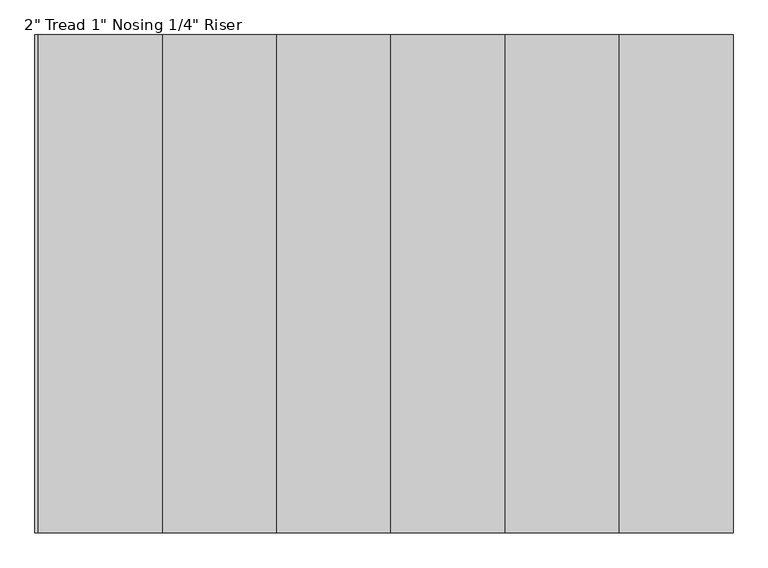
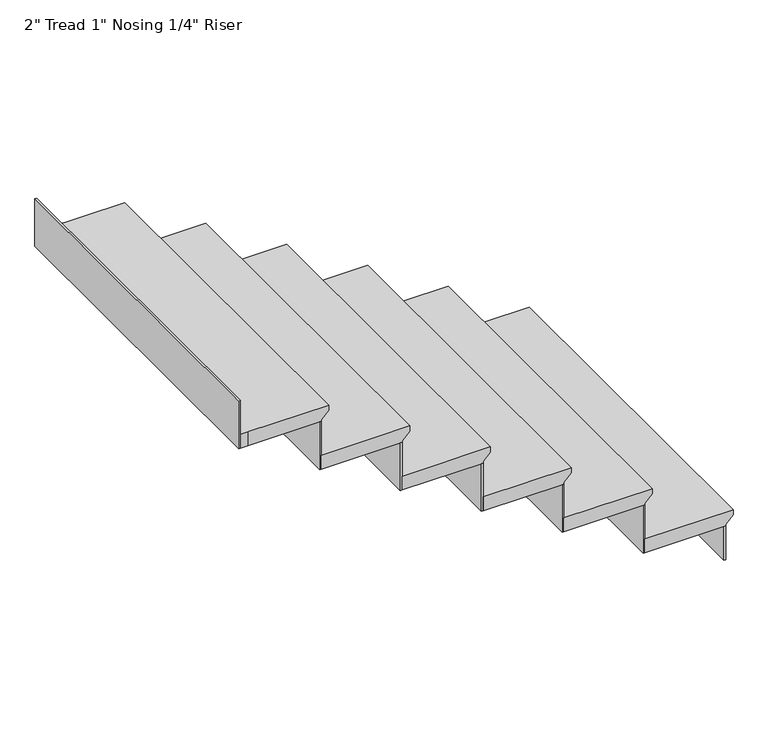
"""IFC4 building model written with IfcOpenShell, lengths in millimetres: stair flight geometry."""

import ifcopenshell
import ifcopenshell.guid

model = None  # the IFC model being written
_history = None  # IfcOwnerHistory: only IFC2X3 demands one
_inside = {}  # id of a spatial element -> (the spatial element, [elements in it])
_under = {}  # id of a project, library or spatial element -> (it, [spatial elements below it])
_declared = {}  # id of a project -> (the project, [libraries it declares])
_typed = {}  # id of a type object -> (the type object, [elements of that type])
_made_of = {}  # id of a material, layer set ... -> (it, [elements and type objects made of it])


def new_model(schema):
    """Start an empty IFC model of exactly this schema.

    Asked for "IFC4X3", IfcOpenShell would pick the latest addendum, in which some entities
    have other attributes; the version numbers below select the first issue.
    IFC2X3 requires an IfcOwnerHistory on every rooted entity: one is made here for all.
    """
    global model, _history
    if schema == "IFC4X3":
        model = ifcopenshell.file(schema_version=(4, 3, 0, 0))
    else:
        model = ifcopenshell.file(schema=schema)
    _inside.clear()
    _under.clear()
    _declared.clear()
    _typed.clear()
    _made_of.clear()
    _history = None
    if model.schema == "IFC2X3":
        org = make("IfcOrganization", Name="unknown")
        user = make(
            "IfcPersonAndOrganization",
            ThePerson=make("IfcPerson", FamilyName="unknown"),
            TheOrganization=org,
        )
        app = make(
            "IfcApplication",
            ApplicationDeveloper=org,
            Version="unknown",
            ApplicationFullName="unknown",
            ApplicationIdentifier="unknown",
        )
        _history = make(
            "IfcOwnerHistory",
            OwningUser=user,
            OwningApplication=app,
            ChangeAction="ADDED",
            CreationDate=0,
        )
    return model


def make(cls, **values):
    """One entity of the class cls with the attributes given. An attribute that is None is left unset."""
    return model.create_entity(
        cls, **{name: value for name, value in values.items() if value is not None}
    )


def rooted(cls, **values):
    """An entity with a GlobalId (a new one), such as an element, a storey or a relation."""
    return make(cls, GlobalId=ifcopenshell.guid.new(), OwnerHistory=_history, **values)


def si_unit(unit_type, name, prefix=None):
    """IfcSIUnit, for example si_unit("LENGTHUNIT", "METRE", prefix="MILLI")."""
    return make("IfcSIUnit", UnitType=unit_type, Prefix=prefix, Name=name)


def assignment(units):
    """IfcUnitAssignment: the units of a project."""
    return None if units is None else make("IfcUnitAssignment", Units=units)


def point(xyz):
    """IfcCartesianPoint."""
    return None if xyz is None else make("IfcCartesianPoint", Coordinates=xyz)


def direction(xyz):
    """IfcDirection."""
    return None if xyz is None else make("IfcDirection", DirectionRatios=xyz)


def frame(location, z_axis=None, x_axis=None):
    """IfcAxis2Placement3D, a coordinate frame: its origin and axes. An axis left out is left unset."""
    return make(
        "IfcAxis2Placement3D",
        Location=point(location),
        Axis=direction(z_axis),
        RefDirection=direction(x_axis),
    )


def origin():
    """The frame at (0, 0, 0) with its axes left unset."""
    return frame((0.0, 0.0, 0.0))


def place(relative_to, where):
    """IfcLocalPlacement: puts the frame where relative to a parent placement (None: the world)."""
    return make(
        "IfcLocalPlacement", PlacementRelTo=relative_to, RelativePlacement=where
    )


def context(
    kind, dimensions, precision=None, world=None, true_north=None, identifier=None
):
    """IfcGeometricRepresentationContext, for example the 3D "Model" context."""
    return make(
        "IfcGeometricRepresentationContext",
        ContextIdentifier=identifier,
        ContextType=kind,
        CoordinateSpaceDimension=dimensions,
        Precision=precision,
        WorldCoordinateSystem=world,
        TrueNorth=true_north,
    )


def project(units=None, contexts=None):
    """IfcProject with its units and contexts."""
    return rooted(
        "IfcProject",
        Name="project",
        RepresentationContexts=contexts,
        UnitsInContext=assignment(units),
    )


def spatial(cls, under=None, at=None, **own):
    """A site, building, storey or space (cls), placed at a placement, below another one or the project."""
    s = rooted(cls, ObjectPlacement=at, **own)
    if under is not None:
        _under.setdefault(under.id(), (under, []))[1].append(s)
    return s


def faces_of(points, faces, orient=None, outer=None):
    """IfcFace entities. A face is a list of loops; a loop is a list of indices into points, from 0.

    orient and outer hold one flag for each loop. By default every Orientation is true, the
    first loop of a face is its IfcFaceOuterBound and the others are IfcFaceBound.
    """
    made = []
    for i, loops in enumerate(faces):
        bounds = []
        for j, loop in enumerate(loops):
            is_outer = j == 0 if outer is None else outer[i][j]
            bounds.append(
                make(
                    "IfcFaceOuterBound" if is_outer else "IfcFaceBound",
                    Bound=make("IfcPolyLoop", Polygon=[points[k] for k in loop]),
                    Orientation=True if orient is None else orient[i][j],
                )
            )
        made.append(make("IfcFace", Bounds=bounds))
    return made


def faceted_brep(points, faces, orient=None, outer=None, voids=None):
    """IfcFacetedBrep: a solid bounded by flat faces; with voids (closed shells), ...WithVoids."""
    shared = [point(p) for p in points]
    hull = make("IfcClosedShell", CfsFaces=faces_of(shared, faces, orient, outer))
    if voids is None:
        return make("IfcFacetedBrep", Outer=hull)
    return make(
        "IfcFacetedBrepWithVoids",
        Outer=hull,
        Voids=[
            make(cls, CfsFaces=faces_of(shared, fs, o, b)) for cls, fs, o, b in voids
        ],
    )


def shape(context_of_items, identifier, shape_type, items):
    """IfcShapeRepresentation: the items that make up one representation, for example the "Body"."""
    return make(
        "IfcShapeRepresentation",
        ContextOfItems=context_of_items,
        RepresentationIdentifier=identifier,
        RepresentationType=shape_type,
        Items=items,
    )


def source(mapping_origin, context_of_items, identifier, shape_type, items):
    """IfcRepresentationMap: a shape defined once, which mapped items show again and again."""
    return make(
        "IfcRepresentationMap",
        MappingOrigin=mapping_origin,
        MappedRepresentation=shape(context_of_items, identifier, shape_type, items),
    )


def transform(
    local_origin,
    x_axis=None,
    y_axis=None,
    z_axis=None,
    scale=None,
    scale2=None,
    scale3=None,
    uniform=True,
):
    """IfcCartesianTransformationOperator3D, or its non-uniform kind. x_axis, y_axis, z_axis: its Axis1, 2, 3."""
    if uniform:
        return make(
            "IfcCartesianTransformationOperator3D",
            Axis1=direction(x_axis),
            Axis2=direction(y_axis),
            LocalOrigin=point(local_origin),
            Scale=scale,
            Axis3=direction(z_axis),
        )
    return make(
        "IfcCartesianTransformationOperator3DnonUniform",
        Axis1=direction(x_axis),
        Axis2=direction(y_axis),
        LocalOrigin=point(local_origin),
        Scale=scale,
        Axis3=direction(z_axis),
        Scale2=scale2,
        Scale3=scale3,
    )


def mapped(mapping_source, mapping_target):
    """IfcMappedItem: shows the shape of a source again, moved by a transform."""
    return make(
        "IfcMappedItem", MappingSource=mapping_source, MappingTarget=mapping_target
    )


def made_of(thing, what):
    """Note that an element or type object is made of a material, layer set ...; save() writes the relation."""
    if what is not None:
        _made_of.setdefault(what.id(), (what, []))[1].append(thing)
    return thing


def element(
    cls,
    number,
    at=None,
    inside=None,
    cuts=None,
    type_object=None,
    material=None,
    context=None,
    identifier="Body",
    shape_type=None,
    held_by="IfcProductDefinitionShape",
    body=None,
    shapes=None,
    **own,
):
    """One element of the class cls, such as IfcWall. Its Tag is "e" and its number.

    at: its placement. inside: the storey or other place that contains it. cuts: it is an
    opening in that element (IfcRelVoidsElement). A single representation is given by context,
    identifier, shape_type and body (its items); several are given by shapes. held_by: the class
    of the entity that holds the representations. save() writes the other relations.
    """
    e = rooted(cls, Tag="e%d" % number, ObjectPlacement=at, **own)
    if body is not None:
        shapes = [shape(context, identifier, shape_type, body)]
    if shapes is not None:
        e.Representation = make(held_by, Representations=shapes)
    if inside is not None:
        _inside.setdefault(inside.id(), (inside, []))[1].append(e)
    if cuts is not None:
        rooted(
            "IfcRelVoidsElement", RelatingBuildingElement=cuts, RelatedOpeningElement=e
        )
    if type_object is not None:
        _typed.setdefault(type_object.id(), (type_object, []))[1].append(e)
    return made_of(e, material)


def aggregate(whole, parts):
    """IfcRelAggregates: a whole, such as a stair, and the parts it consists of."""
    return rooted("IfcRelAggregates", RelatingObject=whole, RelatedObjects=parts)


def save(model, path):
    """Write the relations noted so far, then the file.

    IfcRelAggregates (storeys below a building ...), IfcRelContainedInSpatialStructure (elements
    in a storey), IfcRelDefinesByType, IfcRelAssociatesMaterial and IfcRelDeclares: one each for
    every whole, place, type object, material and project.
    """
    for whole, parts in _under.values():
        aggregate(whole, parts)
    for where, things in _inside.values():
        rooted(
            "IfcRelContainedInSpatialStructure",
            RelatedElements=things,
            RelatingStructure=where,
        )
    for kind, things in _typed.values():
        rooted("IfcRelDefinesByType", RelatedObjects=things, RelatingType=kind)
    for what, things in _made_of.values():
        rooted("IfcRelAssociatesMaterial", RelatedObjects=things, RelatingMaterial=what)
    for by, libraries in _declared.values():
        rooted("IfcRelDeclares", RelatingContext=by, RelatedDefinitions=libraries)
    model.write(path)


def stair_flight_985d9d65(model_context):
    return source(origin(), model_context, "Body", "Brep", [
        faceted_brep([(6344.8601743, -3020.5507921, 155.1214286), (6344.8601743, -3020.5507921, 174.1714286), (6344.8601743, -4239.7507921, 174.1714286), (6344.8601743, -4239.7507921, 155.1214286), (6319.4601743, -3020.5507921, 129.7214286), (6319.4601743, -4239.7507921, 129.7214286), (6040.0601743, -3020.5507921, 174.1714286), (6040.0601743, -4239.7507921, 174.1714286), (6319.4601743, -4239.7507921, 123.3714286), (6040.0601743, -4239.7507921, 123.3714286), (6040.0601743, -3020.5507921, 123.3714286), (6319.4601743, -3020.5507921, 123.3714286)], [[[0, 1, 2, 3]], [[4, 0, 3, 5]], [[2, 1, 6, 7]], [[8, 9, 10, 11]], [[2, 7, 9, 8, 5, 3]], [[8, 11, 4, 5]], [[6, 1, 0, 4, 11, 10]], [[7, 6, 10, 9]]]),
        faceted_brep([(6319.4601743, -3020.5507921, 123.3714286), (6319.4601743, -3020.5507921, 0.0), (6313.1101743, -3020.5507921, 0.0), (6313.1101743, -3020.5507921, 123.3714286), (6319.4601743, -4239.7507921, 123.3714286), (6313.1101743, -4239.7507921, 123.3714286), (6313.1101743, -4239.7507921, 0.0), (6319.4601743, -4239.7507921, 0.0)], [[[0, 1, 2, 3]], [[4, 5, 6, 7]], [[1, 0, 4, 7]], [[2, 1, 7, 6]], [[3, 2, 6, 5]], [[0, 3, 5, 4]]]),
        faceted_brep([(6040.0601743, -3020.5507921, 297.5428571), (6040.0601743, -3020.5507921, 123.3714286), (6033.7101743, -3020.5507921, 123.3714286), (6033.7101743, -3020.5507921, 297.5428571), (6040.0601743, -4239.7507921, 297.5428571), (6033.7101743, -4239.7507921, 297.5428571), (6033.7101743, -4239.7507921, 123.3714286), (6040.0601743, -4239.7507921, 123.3714286)], [[[0, 1, 2, 3]], [[4, 5, 6, 7]], [[1, 0, 4, 7]], [[2, 1, 7, 6]], [[3, 2, 6, 5]], [[0, 3, 5, 4]]]),
        faceted_brep([(6065.4601743, -4239.7507921, 348.3428571), (6065.4601743, -3020.5507921, 348.3428571), (5760.6601743, -3020.5507921, 348.3428571), (5760.6601743, -4239.7507921, 348.3428571), (6040.0601743, -4239.7507921, 297.5428571), (5760.6601743, -4239.7507921, 297.5428571), (5760.6601743, -3020.5507921, 297.5428571), (6040.0601743, -3020.5507921, 297.5428571), (6040.0601743, -4239.7507921, 303.8928571), (6065.4601743, -4239.7507921, 329.2928571), (6040.0601743, -3020.5507921, 303.8928571), (6065.4601743, -3020.5507921, 329.2928571)], [[[0, 1, 2, 3]], [[4, 5, 6, 7]], [[0, 3, 5, 4, 8, 9]], [[4, 7, 10, 8]], [[2, 1, 11, 10, 7, 6]], [[3, 2, 6, 5]], [[11, 1, 0, 9]], [[10, 11, 9, 8]]]),
        faceted_brep([(5760.6601743, -3020.5507921, 471.7142857), (5760.6601743, -3020.5507921, 297.5428571), (5754.3101743, -3020.5507921, 297.5428571), (5754.3101743, -3020.5507921, 471.7142857), (5760.6601743, -4239.7507921, 471.7142857), (5754.3101743, -4239.7507921, 471.7142857), (5754.3101743, -4239.7507921, 297.5428571), (5760.6601743, -4239.7507921, 297.5428571)], [[[0, 1, 2, 3]], [[4, 5, 6, 7]], [[1, 0, 4, 7]], [[2, 1, 7, 6]], [[3, 2, 6, 5]], [[0, 3, 5, 4]]]),
        faceted_brep([(5786.0601743, -4239.7507921, 522.5142857), (5786.0601743, -3020.5507921, 522.5142857), (5481.2601743, -3020.5507921, 522.5142857), (5481.2601743, -4239.7507921, 522.5142857), (5760.6601743, -4239.7507921, 471.7142857), (5481.2601743, -4239.7507921, 471.7142857), (5481.2601743, -3020.5507921, 471.7142857), (5760.6601743, -3020.5507921, 471.7142857), (5760.6601743, -4239.7507921, 478.0642857), (5786.0601743, -4239.7507921, 503.4642857), (5760.6601743, -3020.5507921, 478.0642857), (5786.0601743, -3020.5507921, 503.4642857)], [[[0, 1, 2, 3]], [[4, 5, 6, 7]], [[0, 3, 5, 4, 8, 9]], [[4, 7, 10, 8]], [[2, 1, 11, 10, 7, 6]], [[3, 2, 6, 5]], [[11, 1, 0, 9]], [[10, 11, 9, 8]]]),
        faceted_brep([(5481.2601743, -3020.5507921, 645.8857143), (5481.2601743, -3020.5507921, 471.7142857), (5474.9101743, -3020.5507921, 471.7142857), (5474.9101743, -3020.5507921, 645.8857143), (5481.2601743, -4239.7507921, 645.8857143), (5474.9101743, -4239.7507921, 645.8857143), (5474.9101743, -4239.7507921, 471.7142857), (5481.2601743, -4239.7507921, 471.7142857)], [[[0, 1, 2, 3]], [[4, 5, 6, 7]], [[1, 0, 4, 7]], [[2, 1, 7, 6]], [[3, 2, 6, 5]], [[0, 3, 5, 4]]]),
        faceted_brep([(5506.6601743, -4239.7507921, 696.6857143), (5506.6601743, -3020.5507921, 696.6857143), (5201.8601743, -3020.5507921, 696.6857143), (5201.8601743, -4239.7507921, 696.6857143), (5481.2601743, -4239.7507921, 645.8857143), (5201.8601743, -4239.7507921, 645.8857143), (5201.8601743, -3020.5507921, 645.8857143), (5481.2601743, -3020.5507921, 645.8857143), (5481.2601743, -4239.7507921, 652.2357143), (5506.6601743, -4239.7507921, 677.6357143), (5481.2601743, -3020.5507921, 652.2357143), (5506.6601743, -3020.5507921, 677.6357143)], [[[0, 1, 2, 3]], [[4, 5, 6, 7]], [[0, 3, 5, 4, 8, 9]], [[4, 7, 10, 8]], [[2, 1, 11, 10, 7, 6]], [[3, 2, 6, 5]], [[11, 1, 0, 9]], [[10, 11, 9, 8]]]),
        faceted_brep([(5201.8601743, -3020.5507921, 820.0571429), (5201.8601743, -3020.5507921, 645.8857143), (5195.5101743, -3020.5507921, 645.8857143), (5195.5101743, -3020.5507921, 820.0571429), (5201.8601743, -4239.7507921, 820.0571429), (5195.5101743, -4239.7507921, 820.0571429), (5195.5101743, -4239.7507921, 645.8857143), (5201.8601743, -4239.7507921, 645.8857143)], [[[0, 1, 2, 3]], [[4, 5, 6, 7]], [[1, 0, 4, 7]], [[2, 1, 7, 6]], [[3, 2, 6, 5]], [[0, 3, 5, 4]]]),
        faceted_brep([(5227.2601743, -4239.7507921, 870.8571429), (5227.2601743, -3020.5507921, 870.8571429), (4922.4601743, -3020.5507921, 870.8571429), (4922.4601743, -4239.7507921, 870.8571429), (5201.8601743, -4239.7507921, 820.0571429), (4922.4601743, -4239.7507921, 820.0571429), (4922.4601743, -3020.5507921, 820.0571429), (5201.8601743, -3020.5507921, 820.0571429), (5201.8601743, -4239.7507921, 826.4071429), (5227.2601743, -4239.7507921, 851.8071429), (5201.8601743, -3020.5507921, 826.4071429), (5227.2601743, -3020.5507921, 851.8071429)], [[[0, 1, 2, 3]], [[4, 5, 6, 7]], [[0, 3, 5, 4, 8, 9]], [[4, 7, 10, 8]], [[2, 1, 11, 10, 7, 6]], [[3, 2, 6, 5]], [[11, 1, 0, 9]], [[10, 11, 9, 8]]]),
        faceted_brep([(4922.4601743, -3020.5507921, 994.2285714), (4922.4601743, -3020.5507921, 820.0571429), (4916.1101743, -3020.5507921, 820.0571429), (4916.1101743, -3020.5507921, 994.2285714), (4922.4601743, -4239.7507921, 994.2285714), (4916.1101743, -4239.7507921, 994.2285714), (4916.1101743, -4239.7507921, 820.0571429), (4922.4601743, -4239.7507921, 820.0571429)], [[[0, 1, 2, 3]], [[4, 5, 6, 7]], [[1, 0, 4, 7]], [[2, 1, 7, 6]], [[3, 2, 6, 5]], [[0, 3, 5, 4]]]),
        faceted_brep([(4643.0601743, -3020.5507921, 1168.4), (4643.0601743, -3020.5507921, 994.2285714), (4636.7101743, -3020.5507921, 994.2285714), (4636.7101743, -3020.5507921, 1168.4), (4643.0601743, -4239.7507921, 1168.4), (4636.7101743, -4239.7507921, 1168.4), (4636.7101743, -4239.7507921, 994.2285714), (4643.0601743, -4239.7507921, 994.2285714)], [[[0, 1, 2, 3]], [[4, 5, 6, 7]], [[1, 0, 4, 7]], [[2, 1, 7, 6]], [[3, 2, 6, 5]], [[0, 3, 5, 4]]]),
        faceted_brep([(4643.0601743, -4239.7507921, 1045.0285714), (4668.4601743, -4239.7507921, 1045.0285714), (4947.8601743, -4239.7507921, 1045.0285714), (4947.8601743, -3020.5507921, 1045.0285714), (4668.4601743, -3020.5507921, 1045.0285714), (4643.0601743, -3020.5507921, 1045.0285714), (4668.4601743, -4239.7507921, 994.2285714), (4643.0601743, -4239.7507921, 994.2285714), (4643.0601743, -3020.5507921, 994.2285714), (4668.4601743, -3020.5507921, 994.2285714), (4922.4601743, -3020.5507921, 994.2285714), (4922.4601743, -4239.7507921, 994.2285714), (4922.4601743, -3020.5507921, 1000.5785714), (4922.4601743, -4239.7507921, 1000.5785714), (4947.8601743, -3020.5507921, 1025.9785714), (4947.8601743, -4239.7507921, 1025.9785714)], [[[0, 1, 2, 3, 4, 5]], [[6, 7, 8, 9, 10, 11]], [[1, 0, 7, 6]], [[11, 10, 12, 13]], [[4, 3, 14, 12, 10, 9]], [[5, 4, 9, 8]], [[0, 5, 8, 7]], [[14, 3, 2, 15]], [[12, 14, 15, 13]], [[2, 1, 6, 11, 13, 15]]]),
    ])


if __name__ == "__main__":
    model = new_model("IFC4")
    model_context = context("Model", 3, world=origin())
    ifc_project = project(units=[si_unit("LENGTHUNIT", "METRE", prefix="MILLI")], contexts=[model_context])
    site = spatial("IfcSite", under=ifc_project)
    building = spatial("IfcBuilding", under=site)
    placement = place(None, origin())
    stair_flight_shape = stair_flight_985d9d65(model_context)
    element("IfcStairFlight", 1, ObjectType="2\" Tread 1\" Nosing 1/4\" Riser", at=placement, inside=building, context=model_context, shape_type="MappedRepresentation", body=[
        mapped(stair_flight_shape, transform((0.0, 0.0, 0.0), x_axis=(1.0, 0.0, 0.0), y_axis=(0.0, 1.0, 0.0), z_axis=(0.0, 0.0, 1.0))),
    ])
    save(model, "model.ifc")
